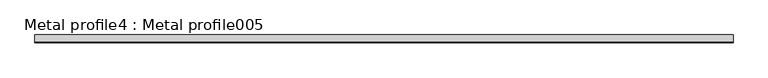
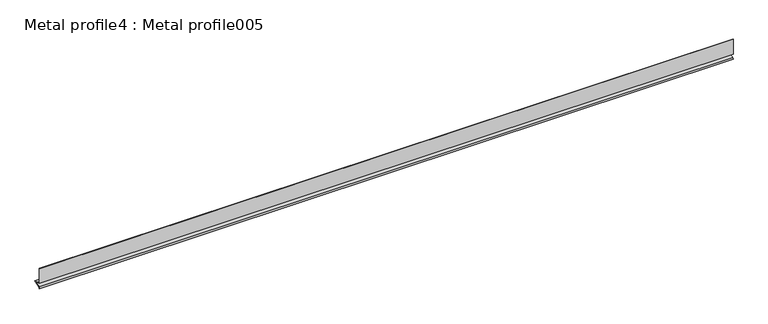
"""IFC4 building model written with IfcOpenShell, lengths in millimetres: proxy geometry, Metal profile4 : Metal profile005."""

from ifc_helpers import new_model, si_unit, frame, origin, place, context, project, spatial, polyline, outline, extrude, source, transform, mapped, element, save


def metal_profile4_metal_profile005_ed59fdcc(model_context):
    return source(origin(), model_context, "Body", "SweptSolid", [
        extrude(outline(polyline([(9752.5625834, 36534.6207792), (9753.5257785, 36539.7355295), (9770.6373811, 36545.2356875), (9752.5625834, 36551.0454439), (9752.5625834, 36596.0356875), (9753.8325834, 36596.0356875), (9753.8325834, 36551.9712232), (9774.7875834, 36545.2356875), (9754.6339669, 36538.7577393), (9753.8106459, 36534.3857476), (9752.5625834, 36534.6207792)])), frame((3694.2883192, 0.0, 0.0), z_axis=(1.0, 0.0, 0.0), x_axis=(0.0, 1.0, 0.0)), (0.0, 0.0, 1.0), 2000.0),
    ])


if __name__ == "__main__":
    model = new_model("IFC4")
    model_context = context("Model", 3, world=origin())
    ifc_project = project(units=[si_unit("LENGTHUNIT", "METRE", prefix="MILLI")], contexts=[model_context])
    site = spatial("IfcSite", under=ifc_project)
    building = spatial("IfcBuilding", under=site)
    placement = place(None, origin())
    metal_profile4_metal_profile005_shape = metal_profile4_metal_profile005_ed59fdcc(model_context)
    element("IfcBuildingElementProxy", 1, Name="Metal profile4 : Metal profile005", ObjectType="Metal profile4 : Metal profile005", at=placement, inside=building, context=model_context, shape_type="MappedRepresentation", body=[
        mapped(metal_profile4_metal_profile005_shape, transform((0.0, 0.0, 0.0), x_axis=(1.0, 0.0, 0.0), y_axis=(0.0, 1.0, 0.0), z_axis=(0.0, 0.0, 1.0))),
    ])
    save(model, "model.ifc")

# Revit data of these elements
# Type "Metal profile4 : Metal profile005"
#   NameOverride = "Metal profile005"
# Element 1 (IfcBuildingElementProxy, "Metal profile4 : Metal profile005")
#   Materials on its faces: "16 GA. COPPER WEEP SCREED W/ MIN 3 1/2\" ATTACHMENT FLANGE - LAP UNDERLAYMENT OVER WEED SCREED"
# Materials
#   "16 GA. COPPER WEEP SCREED W/ MIN 3 1/2\" ATTACHMENT FLANGE - LAP UNDERLAYMENT OVER WEED SCREED": class "Unassigned", colour RGB 251 232 155, transparency 0, Cost = 0
